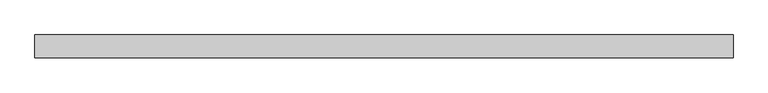
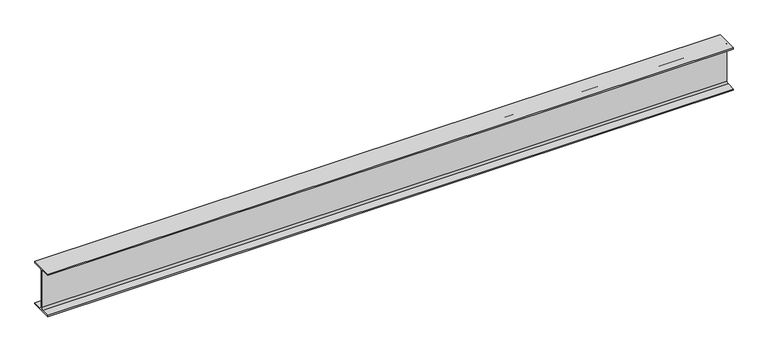
"""IFC4 building model written with IfcOpenShell, lengths in millimetres: beam geometry, 0912_Steel Framing_H-KSD3502 : H_SB_AR_S02_H-300x150x6.5x9_Stair."""

import ifcopenshell
import ifcopenshell.guid

model = None  # the IFC model being written
_history = None  # IfcOwnerHistory: only IFC2X3 demands one
_inside = {}  # id of a spatial element -> (the spatial element, [elements in it])
_under = {}  # id of a project, library or spatial element -> (it, [spatial elements below it])
_declared = {}  # id of a project -> (the project, [libraries it declares])
_typed = {}  # id of a type object -> (the type object, [elements of that type])
_made_of = {}  # id of a material, layer set ... -> (it, [elements and type objects made of it])


def new_model(schema):
    """Start an empty IFC model of exactly this schema.

    Asked for "IFC4X3", IfcOpenShell would pick the latest addendum, in which some entities
    have other attributes; the version numbers below select the first issue.
    IFC2X3 requires an IfcOwnerHistory on every rooted entity: one is made here for all.
    """
    global model, _history
    if schema == "IFC4X3":
        model = ifcopenshell.file(schema_version=(4, 3, 0, 0))
    else:
        model = ifcopenshell.file(schema=schema)
    _inside.clear()
    _under.clear()
    _declared.clear()
    _typed.clear()
    _made_of.clear()
    _history = None
    if model.schema == "IFC2X3":
        org = make("IfcOrganization", Name="unknown")
        user = make(
            "IfcPersonAndOrganization",
            ThePerson=make("IfcPerson", FamilyName="unknown"),
            TheOrganization=org,
        )
        app = make(
            "IfcApplication",
            ApplicationDeveloper=org,
            Version="unknown",
            ApplicationFullName="unknown",
            ApplicationIdentifier="unknown",
        )
        _history = make(
            "IfcOwnerHistory",
            OwningUser=user,
            OwningApplication=app,
            ChangeAction="ADDED",
            CreationDate=0,
        )
    return model


def make(cls, **values):
    """One entity of the class cls with the attributes given. An attribute that is None is left unset."""
    return model.create_entity(
        cls, **{name: value for name, value in values.items() if value is not None}
    )


def rooted(cls, **values):
    """An entity with a GlobalId (a new one), such as an element, a storey or a relation."""
    return make(cls, GlobalId=ifcopenshell.guid.new(), OwnerHistory=_history, **values)


def si_unit(unit_type, name, prefix=None):
    """IfcSIUnit, for example si_unit("LENGTHUNIT", "METRE", prefix="MILLI")."""
    return make("IfcSIUnit", UnitType=unit_type, Prefix=prefix, Name=name)


def assignment(units):
    """IfcUnitAssignment: the units of a project."""
    return None if units is None else make("IfcUnitAssignment", Units=units)


def point(xyz):
    """IfcCartesianPoint."""
    return None if xyz is None else make("IfcCartesianPoint", Coordinates=xyz)


def direction(xyz):
    """IfcDirection."""
    return None if xyz is None else make("IfcDirection", DirectionRatios=xyz)


def frame(location, z_axis=None, x_axis=None):
    """IfcAxis2Placement3D, a coordinate frame: its origin and axes. An axis left out is left unset."""
    return make(
        "IfcAxis2Placement3D",
        Location=point(location),
        Axis=direction(z_axis),
        RefDirection=direction(x_axis),
    )


def frame_2d(location, x_axis=None):
    """IfcAxis2Placement2D, a coordinate frame in the plane: its origin and x axis."""
    return make(
        "IfcAxis2Placement2D", Location=point(location), RefDirection=direction(x_axis)
    )


def origin():
    """The frame at (0, 0, 0) with its axes left unset."""
    return frame((0.0, 0.0, 0.0))


def place(relative_to, where):
    """IfcLocalPlacement: puts the frame where relative to a parent placement (None: the world)."""
    return make(
        "IfcLocalPlacement", PlacementRelTo=relative_to, RelativePlacement=where
    )


def context(
    kind, dimensions, precision=None, world=None, true_north=None, identifier=None
):
    """IfcGeometricRepresentationContext, for example the 3D "Model" context."""
    return make(
        "IfcGeometricRepresentationContext",
        ContextIdentifier=identifier,
        ContextType=kind,
        CoordinateSpaceDimension=dimensions,
        Precision=precision,
        WorldCoordinateSystem=world,
        TrueNorth=true_north,
    )


def project(units=None, contexts=None):
    """IfcProject with its units and contexts."""
    return rooted(
        "IfcProject",
        Name="project",
        RepresentationContexts=contexts,
        UnitsInContext=assignment(units),
    )


def spatial(cls, under=None, at=None, **own):
    """A site, building, storey or space (cls), placed at a placement, below another one or the project."""
    s = rooted(cls, ObjectPlacement=at, **own)
    if under is not None:
        _under.setdefault(under.id(), (under, []))[1].append(s)
    return s


def polyline(points):
    """IfcPolyline through the points."""
    return make("IfcPolyline", Points=[point(p) for p in points])


def circle_curve(where, radius):
    """IfcCircle in the frame where."""
    return make("IfcCircle", Position=where, Radius=radius)


def trimmed(basis, trim1, trim2, sense, master):
    """IfcTrimmedCurve: the piece of a basis curve between two trims."""
    return make(
        "IfcTrimmedCurve",
        BasisCurve=basis,
        Trim1=trim1,
        Trim2=trim2,
        SenseAgreement=sense,
        MasterRepresentation=master,
    )


def segment(curve, same_sense, transition):
    """IfcCompositeCurveSegment."""
    return make(
        "IfcCompositeCurveSegment",
        Transition=transition,
        SameSense=same_sense,
        ParentCurve=curve,
    )


def composite_curve(segments, self_intersect=None):
    """IfcCompositeCurve: segments joined end to end."""
    return make("IfcCompositeCurve", Segments=segments, SelfIntersect=self_intersect)


def outline(outer, holes=None, kind="AREA"):
    """IfcArbitraryClosedProfileDef: a profile drawn as a closed curve; with holes, ...WithVoids."""
    if holes is None:
        return make("IfcArbitraryClosedProfileDef", ProfileType=kind, OuterCurve=outer)
    return make(
        "IfcArbitraryProfileDefWithVoids",
        ProfileType=kind,
        OuterCurve=outer,
        InnerCurves=holes,
    )


def extrude(swept, where, along, depth):
    """IfcExtrudedAreaSolid: the profile swept, set in the frame where, extruded along a direction by depth."""
    return make(
        "IfcExtrudedAreaSolid",
        SweptArea=swept,
        Position=where,
        ExtrudedDirection=direction(along),
        Depth=depth,
    )


def shape(context_of_items, identifier, shape_type, items):
    """IfcShapeRepresentation: the items that make up one representation, for example the "Body"."""
    return make(
        "IfcShapeRepresentation",
        ContextOfItems=context_of_items,
        RepresentationIdentifier=identifier,
        RepresentationType=shape_type,
        Items=items,
    )


def source(mapping_origin, context_of_items, identifier, shape_type, items):
    """IfcRepresentationMap: a shape defined once, which mapped items show again and again."""
    return make(
        "IfcRepresentationMap",
        MappingOrigin=mapping_origin,
        MappedRepresentation=shape(context_of_items, identifier, shape_type, items),
    )


def transform(
    local_origin,
    x_axis=None,
    y_axis=None,
    z_axis=None,
    scale=None,
    scale2=None,
    scale3=None,
    uniform=True,
):
    """IfcCartesianTransformationOperator3D, or its non-uniform kind. x_axis, y_axis, z_axis: its Axis1, 2, 3."""
    if uniform:
        return make(
            "IfcCartesianTransformationOperator3D",
            Axis1=direction(x_axis),
            Axis2=direction(y_axis),
            LocalOrigin=point(local_origin),
            Scale=scale,
            Axis3=direction(z_axis),
        )
    return make(
        "IfcCartesianTransformationOperator3DnonUniform",
        Axis1=direction(x_axis),
        Axis2=direction(y_axis),
        LocalOrigin=point(local_origin),
        Scale=scale,
        Axis3=direction(z_axis),
        Scale2=scale2,
        Scale3=scale3,
    )


def mapped(mapping_source, mapping_target):
    """IfcMappedItem: shows the shape of a source again, moved by a transform."""
    return make(
        "IfcMappedItem", MappingSource=mapping_source, MappingTarget=mapping_target
    )


def made_of(thing, what):
    """Note that an element or type object is made of a material, layer set ...; save() writes the relation."""
    if what is not None:
        _made_of.setdefault(what.id(), (what, []))[1].append(thing)
    return thing


def element(
    cls,
    number,
    at=None,
    inside=None,
    cuts=None,
    type_object=None,
    material=None,
    context=None,
    identifier="Body",
    shape_type=None,
    held_by="IfcProductDefinitionShape",
    body=None,
    shapes=None,
    **own,
):
    """One element of the class cls, such as IfcWall. Its Tag is "e" and its number.

    at: its placement. inside: the storey or other place that contains it. cuts: it is an
    opening in that element (IfcRelVoidsElement). A single representation is given by context,
    identifier, shape_type and body (its items); several are given by shapes. held_by: the class
    of the entity that holds the representations. save() writes the other relations.
    """
    e = rooted(cls, Tag="e%d" % number, ObjectPlacement=at, **own)
    if body is not None:
        shapes = [shape(context, identifier, shape_type, body)]
    if shapes is not None:
        e.Representation = make(held_by, Representations=shapes)
    if inside is not None:
        _inside.setdefault(inside.id(), (inside, []))[1].append(e)
    if cuts is not None:
        rooted(
            "IfcRelVoidsElement", RelatingBuildingElement=cuts, RelatedOpeningElement=e
        )
    if type_object is not None:
        _typed.setdefault(type_object.id(), (type_object, []))[1].append(e)
    return made_of(e, material)


def aggregate(whole, parts):
    """IfcRelAggregates: a whole, such as a stair, and the parts it consists of."""
    return rooted("IfcRelAggregates", RelatingObject=whole, RelatedObjects=parts)


def save(model, path):
    """Write the relations noted so far, then the file.

    IfcRelAggregates (storeys below a building ...), IfcRelContainedInSpatialStructure (elements
    in a storey), IfcRelDefinesByType, IfcRelAssociatesMaterial and IfcRelDeclares: one each for
    every whole, place, type object, material and project.
    """
    for whole, parts in _under.values():
        aggregate(whole, parts)
    for where, things in _inside.values():
        rooted(
            "IfcRelContainedInSpatialStructure",
            RelatedElements=things,
            RelatingStructure=where,
        )
    for kind, things in _typed.values():
        rooted("IfcRelDefinesByType", RelatedObjects=things, RelatingType=kind)
    for what, things in _made_of.values():
        rooted("IfcRelAssociatesMaterial", RelatedObjects=things, RelatingMaterial=what)
    for by, libraries in _declared.values():
        rooted("IfcRelDeclares", RelatingContext=by, RelatedDefinitions=libraries)
    model.write(path)


def beam_4b5297f3(model_context):
    return source(origin(), model_context, "Body", "SweptSolid", [
        extrude(outline(composite_curve([segment(polyline([(75.0, -141.0), (75.0, -150.0), (-75.0, -150.0), (-75.0, -141.0), (-16.25, -141.0)]), True, "CONTINUOUS"), segment(trimmed(circle_curve(frame_2d((-16.25, -128.0)), 13.0), [point((-16.25, -141.0))], [point((-3.25, -128.0))], True, "CARTESIAN"), True, "CONTINUOUS"), segment(polyline([(-3.25, -128.0), (-3.25, 128.0)]), True, "CONTINUOUS"), segment(trimmed(circle_curve(frame_2d((-16.25, 128.0)), 13.0), [point((-3.25, 128.0))], [point((-16.25, 141.0))], True, "CARTESIAN"), True, "CONTINUOUS"), segment(polyline([(-16.25, 141.0), (-75.0, 141.0), (-75.0, 150.0), (75.0, 150.0), (75.0, 141.0), (16.25, 141.0)]), True, "CONTINUOUS"), segment(trimmed(circle_curve(frame_2d((16.25, 128.0)), 13.0), [point((16.25, 141.0))], [point((3.25, 128.0))], True, "CARTESIAN"), True, "CONTINUOUS"), segment(polyline([(3.25, 128.0), (3.25, -128.0)]), True, "CONTINUOUS"), segment(trimmed(circle_curve(frame_2d((16.25, -128.0)), 13.0), [point((3.25, -128.0))], [point((16.25, -141.0))], True, "CARTESIAN"), True, "CONTINUOUS"), segment(polyline([(16.25, -141.0), (75.0, -141.0)]), True, "CONTINUOUS")], self_intersect=False)), frame((-2287.3, 0.0, 0.0), z_axis=(1.0, 0.0, 0.0), x_axis=(0.0, 1.0, 0.0)), (0.0, 0.0, 1.0), 4574.6),
    ])


if __name__ == "__main__":
    model = new_model("IFC4")
    model_context = context("Model", 3, world=origin())
    ifc_project = project(units=[si_unit("LENGTHUNIT", "METRE", prefix="MILLI")], contexts=[model_context])
    site = spatial("IfcSite", under=ifc_project)
    building = spatial("IfcBuilding", under=site)
    placement = place(None, origin())
    beam_shape = beam_4b5297f3(model_context)
    element("IfcBeam", 1, ObjectType="0912_Steel Framing_H-KSD3502 : H_SB_AR_S02_H-300x150x6.5x9_Stair", at=placement, inside=building, context=model_context, shape_type="MappedRepresentation", body=[
        mapped(beam_shape, transform((0.0, 0.0, 0.0), x_axis=(1.0, 0.0, 0.0), y_axis=(0.0, 1.0, 0.0), z_axis=(0.0, 0.0, 1.0))),
    ])
    save(model, "model.ifc")

# Revit data of these elements
# Type "0912_Steel Framing_H-KSD3502 : H_SB_AR_S02_H-300x150x6.5x9_Stair"
#   H_Q'ty Cal Type Tag = "SB-Q2"
#   H_WM Code_1 = "S01AA073-00001 |  | TON | Main Steel Structure Fabrication Work | Shelter/Building | Medium Steel - Standard |  |  |  |  |  |  | Material: (   ) | (90)KG/M>Weight≥(30)KG/M | S01AA073-00001 Main Steel Structure Fabrication Work Shelter/Building Medium Steel - Standard         | - Material: ( ASTM A36 )\n- (90)KG/M>Weight≥(30)KG/M"
#   H_WM Code_2 = "S03AA083-00001 |  | TON | Main Steel Structure Erection Work | Shelter/Building | Medium Steel |  |  |  |  |  |  | Material: (   ) | S03AA083-00001 Main Steel Structure Erection Work Shelter/Building Medium Steel         | - Material: ( ASTM A36 )"
#   H_WM Code_3 = "S01AA009-00001 |  | TON | Main Steel Structure Fabrication Work | Shelter/Building | Plates - Gusset, Stiffener, ETC | Material: (   ) | S01AA009-00001 Main Steel Structure Fabrication Work Shelter/Building Plates - Gusset, Stiffener, ETC         |"
#   H_WM Code_4 = "S41AA051-00001 |  | M2 | Steel Structure Paint Work | Shelter/Building | for Non-Fireproofed Steel Surface |  |  |  |  |  |  | Material: (   ) | S41AA051-00001 Steel Structure Paint Work Shelter/Building for Non-Fireproofed Steel Surface         |"
#   Width = 15.0 cm
#   Web Thickness = 0.65 cm
#   Web Fillet = 1.3 cm
#   Warping Constant = 107000.0 cm⁶
#   W = 0
#   Torsional Moment of Inertia = 9.9539 cm⁴
#   Section Area = 46.78 cm²
#   Plastic Modulus weak axis = 105.0 cm³
#   Plastic Modulus strong axis = 542.0 cm³
#   Perimeter = 1.17 m²/m
#   Nominal Weight = 36.70 kgf/m
#   Moment of Inertia weak axis = 508.00 cm⁴
#   Moment of Inertia strong axis = 7210.00 cm⁴
#   Height = 30.0 cm
#   Flange Thickness = 0.9 cm
#   Elastic Modulus weak axis = 67.7 cm³
#   Elastic Modulus strong axis = 481.0 cm³
#   Centroid Vertical = 15.0 cm
#   Centroid Horizontal = 7.5 cm
#   Ix = 72100000
#   Length [instance default] = 1524 mm
#   Zx = 542000
#   b = 150 mm
#   h = 300 mm
#   r = 13 mm
#   s = 6.5 mm
#   t = 9 mm
#   A = 0.004678 m²
#   Structural Material [instance default] = Steel, 45-345
#   Assembly Code = ""
# Element 1 (IfcBeam, "0912_Steel Framing_H-KSD3502 : H_SB_AR_S02_H-300x150x6.5x9_Stair")
#   Materials on its faces: "Steel, 45-345"
# Materials
#   "Steel, 45-345": class "Metal", colour RGB 189 187 185, transparency 0, Description = "Steel 345 MPa", Cost = 0
